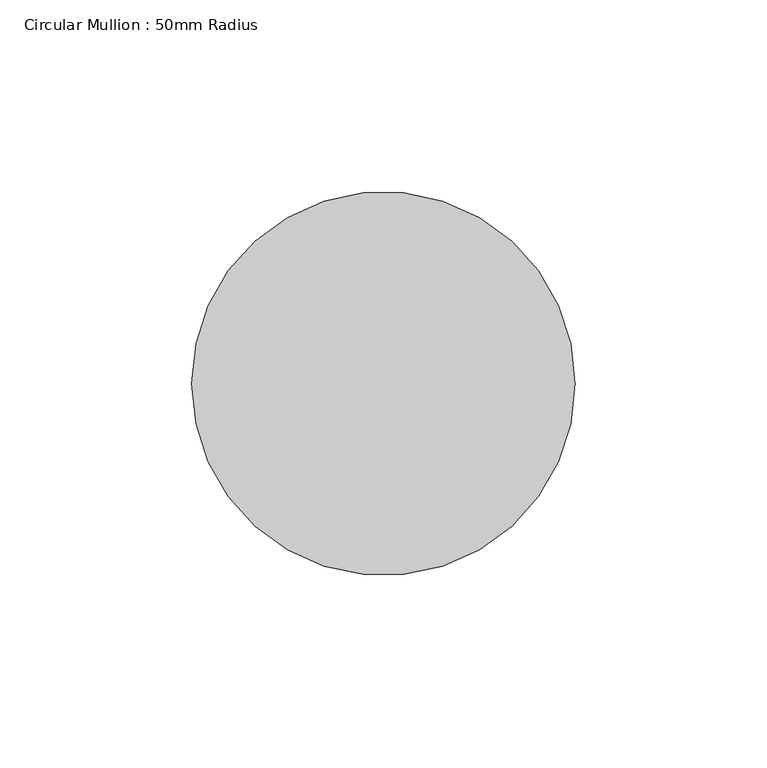
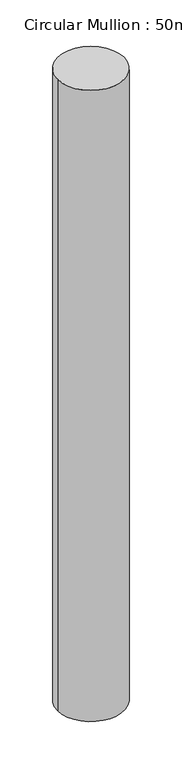
"""IFC4 building model written with IfcOpenShell, lengths in millimetres: member geometry, Circular Mullion : 50mm Radius."""

from ifc_helpers import new_model, si_unit, point, frame, origin, origin_2d, place, context, project, spatial, circle_curve, trimmed, segment, composite_curve, outline, extrude, source, transform, mapped, element, save


def circular_mullion_50mm_radius_20d9eb17(model_context):
    return source(origin(), model_context, "Body", "SweptSolid", [
        extrude(outline(composite_curve([segment(trimmed(circle_curve(origin_2d(), 50.0), [point((50.0, 0.0))], [point((-50.0, 0.0))], False, "CARTESIAN"), True, "CONTINUOUS"), segment(trimmed(circle_curve(origin_2d(), 50.0), [point((-50.0, 0.0))], [point((50.0, 0.0))], False, "CARTESIAN"), True, "CONTINUOUS")], self_intersect=False)), frame((0.0, 0.0, -1003.6484532), z_axis=(0.0, 0.0, 1.0), x_axis=(1.0, 0.0, 0.0)), (0.0, 0.0, 1.0), 1003.6484532),
    ])


if __name__ == "__main__":
    model = new_model("IFC4")
    model_context = context("Model", 3, world=origin())
    ifc_project = project(units=[si_unit("LENGTHUNIT", "METRE", prefix="MILLI")], contexts=[model_context])
    site = spatial("IfcSite", under=ifc_project)
    building = spatial("IfcBuilding", under=site)
    placement = place(None, origin())
    circular_mullion_50mm_radius_shape = circular_mullion_50mm_radius_20d9eb17(model_context)
    element("IfcMember", 1, ObjectType="Circular Mullion : 50mm Radius", at=placement, inside=building, context=model_context, shape_type="MappedRepresentation", body=[
        mapped(circular_mullion_50mm_radius_shape, transform((0.0, 0.0, 0.0), x_axis=(1.0, 0.0, 0.0), y_axis=(0.0, 1.0, 0.0), z_axis=(0.0, 0.0, 1.0))),
    ])
    save(model, "model.ifc")

# Revit data of these elements
# Type "Circular Mullion : 50mm Radius"
#   built-in parameter 1007350 = 0.164042 (stored number, unit not read)
# Element 1 (IfcMember, "Circular Mullion : 50mm Radius")
#   Materials on its faces: "Aluminium"
# Materials
#   "Aluminium": class "Metal", colour RGB 247 247 247, transparency 0, Description = "Aluminium 6061", Cost = 0
